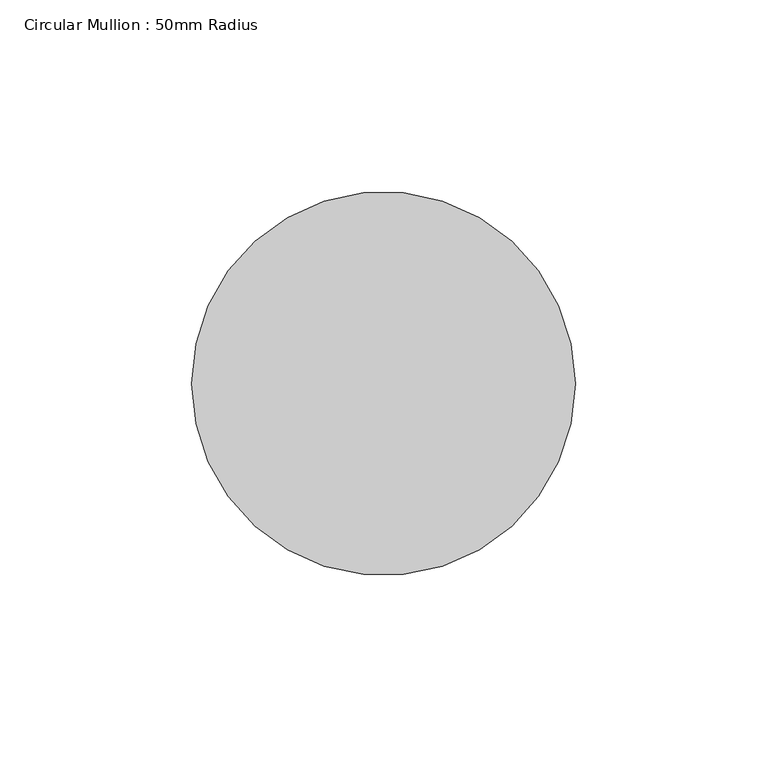
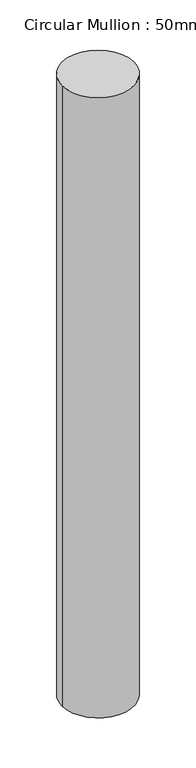
"""IFC4 building model written with IfcOpenShell, lengths in millimetres: member geometry, Circular Mullion : 50mm Radius."""

from ifc_helpers import new_model, si_unit, point, frame, origin, origin_2d, place, context, project, spatial, circle_curve, trimmed, segment, composite_curve, outline, extrude, source, transform, mapped, element, save


def circular_mullion_50mm_radius_9474a210(model_context):
    return source(origin(), model_context, "Body", "SweptSolid", [
        extrude(outline(composite_curve([segment(trimmed(circle_curve(origin_2d(), 50.0), [point((50.0, 0.0))], [point((-50.0, 0.0))], False, "CARTESIAN"), True, "CONTINUOUS"), segment(trimmed(circle_curve(origin_2d(), 50.0), [point((-50.0, 0.0))], [point((50.0, 0.0))], False, "CARTESIAN"), True, "CONTINUOUS")], self_intersect=False)), frame((0.0, 0.0, -914.6272405), z_axis=(0.0, 0.0, 1.0), x_axis=(1.0, 0.0, 0.0)), (0.0, 0.0, 1.0), 914.6272405),
    ])


if __name__ == "__main__":
    model = new_model("IFC4")
    model_context = context("Model", 3, world=origin())
    ifc_project = project(units=[si_unit("LENGTHUNIT", "METRE", prefix="MILLI")], contexts=[model_context])
    site = spatial("IfcSite", under=ifc_project)
    building = spatial("IfcBuilding", under=site)
    placement = place(None, origin())
    circular_mullion_50mm_radius_shape = circular_mullion_50mm_radius_9474a210(model_context)
    element("IfcMember", 1, ObjectType="Circular Mullion : 50mm Radius", at=placement, inside=building, context=model_context, shape_type="MappedRepresentation", body=[
        mapped(circular_mullion_50mm_radius_shape, transform((0.0, 0.0, 0.0), x_axis=(1.0, 0.0, 0.0), y_axis=(0.0, 1.0, 0.0), z_axis=(0.0, 0.0, 1.0))),
    ])
    save(model, "model.ifc")

# Revit data of these elements
# Type "Circular Mullion : 50mm Radius"
#   built-in parameter 1007350 = 0.164042 (stored number, unit not read)
# Element 1 (IfcMember, "Circular Mullion : 50mm Radius")
#   Materials on its faces: "Aluminium"
# Materials
#   "Aluminium": class "Metal", colour RGB 247 247 247, transparency 0, Description = "Aluminium 6061", Cost = 0
